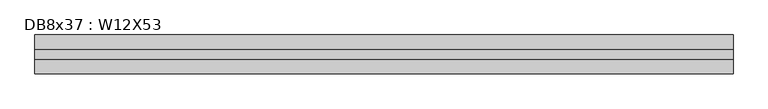
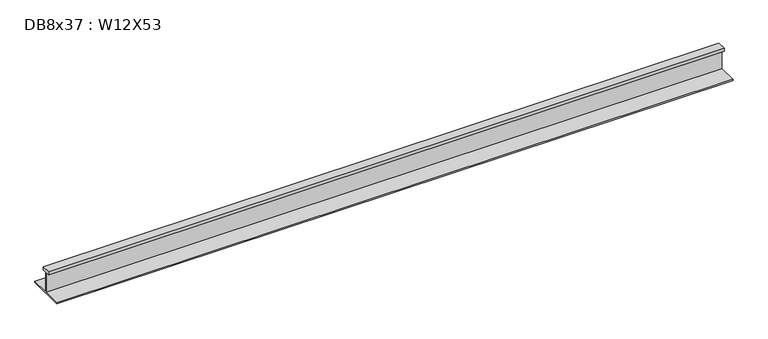
"""IFC4 building model written with IfcOpenShell, lengths in millimetres: beam geometry, DB8x37 : W12X53."""

import ifcopenshell
import ifcopenshell.guid

model = None  # the IFC model being written
_history = None  # IfcOwnerHistory: only IFC2X3 demands one
_inside = {}  # id of a spatial element -> (the spatial element, [elements in it])
_under = {}  # id of a project, library or spatial element -> (it, [spatial elements below it])
_declared = {}  # id of a project -> (the project, [libraries it declares])
_typed = {}  # id of a type object -> (the type object, [elements of that type])
_made_of = {}  # id of a material, layer set ... -> (it, [elements and type objects made of it])


def new_model(schema):
    """Start an empty IFC model of exactly this schema.

    Asked for "IFC4X3", IfcOpenShell would pick the latest addendum, in which some entities
    have other attributes; the version numbers below select the first issue.
    IFC2X3 requires an IfcOwnerHistory on every rooted entity: one is made here for all.
    """
    global model, _history
    if schema == "IFC4X3":
        model = ifcopenshell.file(schema_version=(4, 3, 0, 0))
    else:
        model = ifcopenshell.file(schema=schema)
    _inside.clear()
    _under.clear()
    _declared.clear()
    _typed.clear()
    _made_of.clear()
    _history = None
    if model.schema == "IFC2X3":
        org = make("IfcOrganization", Name="unknown")
        user = make(
            "IfcPersonAndOrganization",
            ThePerson=make("IfcPerson", FamilyName="unknown"),
            TheOrganization=org,
        )
        app = make(
            "IfcApplication",
            ApplicationDeveloper=org,
            Version="unknown",
            ApplicationFullName="unknown",
            ApplicationIdentifier="unknown",
        )
        _history = make(
            "IfcOwnerHistory",
            OwningUser=user,
            OwningApplication=app,
            ChangeAction="ADDED",
            CreationDate=0,
        )
    return model


def make(cls, **values):
    """One entity of the class cls with the attributes given. An attribute that is None is left unset."""
    return model.create_entity(
        cls, **{name: value for name, value in values.items() if value is not None}
    )


def rooted(cls, **values):
    """An entity with a GlobalId (a new one), such as an element, a storey or a relation."""
    return make(cls, GlobalId=ifcopenshell.guid.new(), OwnerHistory=_history, **values)


def si_unit(unit_type, name, prefix=None):
    """IfcSIUnit, for example si_unit("LENGTHUNIT", "METRE", prefix="MILLI")."""
    return make("IfcSIUnit", UnitType=unit_type, Prefix=prefix, Name=name)


def assignment(units):
    """IfcUnitAssignment: the units of a project."""
    return None if units is None else make("IfcUnitAssignment", Units=units)


def point(xyz):
    """IfcCartesianPoint."""
    return None if xyz is None else make("IfcCartesianPoint", Coordinates=xyz)


def direction(xyz):
    """IfcDirection."""
    return None if xyz is None else make("IfcDirection", DirectionRatios=xyz)


def frame(location, z_axis=None, x_axis=None):
    """IfcAxis2Placement3D, a coordinate frame: its origin and axes. An axis left out is left unset."""
    return make(
        "IfcAxis2Placement3D",
        Location=point(location),
        Axis=direction(z_axis),
        RefDirection=direction(x_axis),
    )


def origin():
    """The frame at (0, 0, 0) with its axes left unset."""
    return frame((0.0, 0.0, 0.0))


def place(relative_to, where):
    """IfcLocalPlacement: puts the frame where relative to a parent placement (None: the world)."""
    return make(
        "IfcLocalPlacement", PlacementRelTo=relative_to, RelativePlacement=where
    )


def context(
    kind, dimensions, precision=None, world=None, true_north=None, identifier=None
):
    """IfcGeometricRepresentationContext, for example the 3D "Model" context."""
    return make(
        "IfcGeometricRepresentationContext",
        ContextIdentifier=identifier,
        ContextType=kind,
        CoordinateSpaceDimension=dimensions,
        Precision=precision,
        WorldCoordinateSystem=world,
        TrueNorth=true_north,
    )


def project(units=None, contexts=None):
    """IfcProject with its units and contexts."""
    return rooted(
        "IfcProject",
        Name="project",
        RepresentationContexts=contexts,
        UnitsInContext=assignment(units),
    )


def spatial(cls, under=None, at=None, **own):
    """A site, building, storey or space (cls), placed at a placement, below another one or the project."""
    s = rooted(cls, ObjectPlacement=at, **own)
    if under is not None:
        _under.setdefault(under.id(), (under, []))[1].append(s)
    return s


def polyline(points):
    """IfcPolyline through the points."""
    return make("IfcPolyline", Points=[point(p) for p in points])


def outline(outer, holes=None, kind="AREA"):
    """IfcArbitraryClosedProfileDef: a profile drawn as a closed curve; with holes, ...WithVoids."""
    if holes is None:
        return make("IfcArbitraryClosedProfileDef", ProfileType=kind, OuterCurve=outer)
    return make(
        "IfcArbitraryProfileDefWithVoids",
        ProfileType=kind,
        OuterCurve=outer,
        InnerCurves=holes,
    )


def extrude(swept, where, along, depth):
    """IfcExtrudedAreaSolid: the profile swept, set in the frame where, extruded along a direction by depth."""
    return make(
        "IfcExtrudedAreaSolid",
        SweptArea=swept,
        Position=where,
        ExtrudedDirection=direction(along),
        Depth=depth,
    )


def shape(context_of_items, identifier, shape_type, items):
    """IfcShapeRepresentation: the items that make up one representation, for example the "Body"."""
    return make(
        "IfcShapeRepresentation",
        ContextOfItems=context_of_items,
        RepresentationIdentifier=identifier,
        RepresentationType=shape_type,
        Items=items,
    )


def source(mapping_origin, context_of_items, identifier, shape_type, items):
    """IfcRepresentationMap: a shape defined once, which mapped items show again and again."""
    return make(
        "IfcRepresentationMap",
        MappingOrigin=mapping_origin,
        MappedRepresentation=shape(context_of_items, identifier, shape_type, items),
    )


def transform(
    local_origin,
    x_axis=None,
    y_axis=None,
    z_axis=None,
    scale=None,
    scale2=None,
    scale3=None,
    uniform=True,
):
    """IfcCartesianTransformationOperator3D, or its non-uniform kind. x_axis, y_axis, z_axis: its Axis1, 2, 3."""
    if uniform:
        return make(
            "IfcCartesianTransformationOperator3D",
            Axis1=direction(x_axis),
            Axis2=direction(y_axis),
            LocalOrigin=point(local_origin),
            Scale=scale,
            Axis3=direction(z_axis),
        )
    return make(
        "IfcCartesianTransformationOperator3DnonUniform",
        Axis1=direction(x_axis),
        Axis2=direction(y_axis),
        LocalOrigin=point(local_origin),
        Scale=scale,
        Axis3=direction(z_axis),
        Scale2=scale2,
        Scale3=scale3,
    )


def mapped(mapping_source, mapping_target):
    """IfcMappedItem: shows the shape of a source again, moved by a transform."""
    return make(
        "IfcMappedItem", MappingSource=mapping_source, MappingTarget=mapping_target
    )


def made_of(thing, what):
    """Note that an element or type object is made of a material, layer set ...; save() writes the relation."""
    if what is not None:
        _made_of.setdefault(what.id(), (what, []))[1].append(thing)
    return thing


def element(
    cls,
    number,
    at=None,
    inside=None,
    cuts=None,
    type_object=None,
    material=None,
    context=None,
    identifier="Body",
    shape_type=None,
    held_by="IfcProductDefinitionShape",
    body=None,
    shapes=None,
    **own,
):
    """One element of the class cls, such as IfcWall. Its Tag is "e" and its number.

    at: its placement. inside: the storey or other place that contains it. cuts: it is an
    opening in that element (IfcRelVoidsElement). A single representation is given by context,
    identifier, shape_type and body (its items); several are given by shapes. held_by: the class
    of the entity that holds the representations. save() writes the other relations.
    """
    e = rooted(cls, Tag="e%d" % number, ObjectPlacement=at, **own)
    if body is not None:
        shapes = [shape(context, identifier, shape_type, body)]
    if shapes is not None:
        e.Representation = make(held_by, Representations=shapes)
    if inside is not None:
        _inside.setdefault(inside.id(), (inside, []))[1].append(e)
    if cuts is not None:
        rooted(
            "IfcRelVoidsElement", RelatingBuildingElement=cuts, RelatedOpeningElement=e
        )
    if type_object is not None:
        _typed.setdefault(type_object.id(), (type_object, []))[1].append(e)
    return made_of(e, material)


def aggregate(whole, parts):
    """IfcRelAggregates: a whole, such as a stair, and the parts it consists of."""
    return rooted("IfcRelAggregates", RelatingObject=whole, RelatedObjects=parts)


def save(model, path):
    """Write the relations noted so far, then the file.

    IfcRelAggregates (storeys below a building ...), IfcRelContainedInSpatialStructure (elements
    in a storey), IfcRelDefinesByType, IfcRelAssociatesMaterial and IfcRelDeclares: one each for
    every whole, place, type object, material and project.
    """
    for whole, parts in _under.values():
        aggregate(whole, parts)
    for where, things in _inside.values():
        rooted(
            "IfcRelContainedInSpatialStructure",
            RelatedElements=things,
            RelatingStructure=where,
        )
    for kind, things in _typed.values():
        rooted("IfcRelDefinesByType", RelatedObjects=things, RelatingType=kind)
    for what, things in _made_of.values():
        rooted("IfcRelAssociatesMaterial", RelatedObjects=things, RelatingMaterial=what)
    for by, libraries in _declared.values():
        rooted("IfcRelDeclares", RelatingContext=by, RelatedDefinitions=libraries)
    model.write(path)


def db8x37_w12x53_f22f7946(model_context):
    return source(origin(), model_context, "Body", "SweptSolid", [
        extrude(outline(polyline([(38.1, 145.415), (38.1, 120.015), (2.921, 120.015), (2.921, -48.4505), (152.4, -48.4505), (152.4, -58.1025), (-152.4, -58.1025), (-152.4, -48.4505), (-2.921, -48.4505), (-2.921, 120.015), (-38.1, 120.015), (-38.1, 145.415), (38.1, 145.415)])), frame((-2667.508, 0.0, 0.0), z_axis=(1.0, 0.0, 0.0), x_axis=(0.0, 1.0, 0.0)), (0.0, 0.0, 1.0), 5448.808),
    ])


if __name__ == "__main__":
    model = new_model("IFC4")
    model_context = context("Model", 3, world=origin())
    ifc_project = project(units=[si_unit("LENGTHUNIT", "METRE", prefix="MILLI")], contexts=[model_context])
    site = spatial("IfcSite", under=ifc_project)
    building = spatial("IfcBuilding", under=site)
    placement = place(None, origin())
    db8x37_w12x53_shape = db8x37_w12x53_f22f7946(model_context)
    element("IfcBeam", 1, ObjectType="DB8x37 : W12X53", at=placement, inside=building, context=model_context, shape_type="MappedRepresentation", body=[
        mapped(db8x37_w12x53_shape, transform((0.0, 0.0, 0.0), x_axis=(1.0, 0.0, 0.0), y_axis=(0.0, 1.0, 0.0), z_axis=(0.0, 0.0, 1.0))),
    ])
    save(model, "model.ifc")

# Revit data of these elements
# Type "DB8x37 : W12X53"
#   Assembly Code = "B10"
#   W = 53
#   Length [instance default] = 5' - 0"
#   bf = 0' - 10"
#   d = 1' - 0.1"
#   k = 0' - 1 3/8"
#   k2 = 0' - 0.8"
#   tf = 0' - 0.575"
#   tw = 0' - 0.345"
#   A = 0.108333 SF
#   Structural Material [instance default] = Steel ASTM A992
# Element 1 (IfcBeam, "DB8x37 : W12X53")
#   Materials on its faces: "Steel ASTM A992"
# Materials
#   "Steel ASTM A992": class "Metal", colour RGB 199 199 199, transparency 0, Description = "Structural steel 50ksi", Cost = 0
